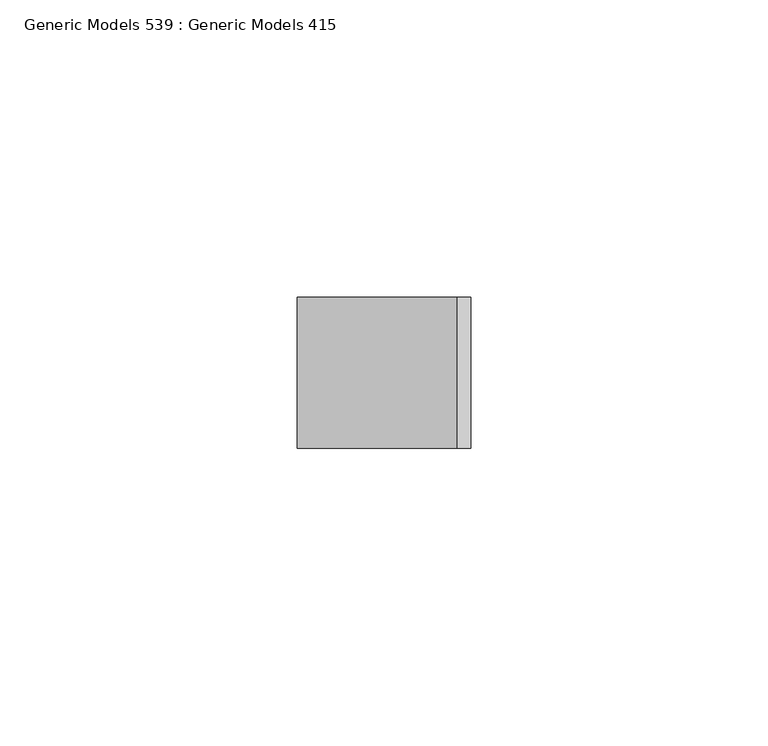
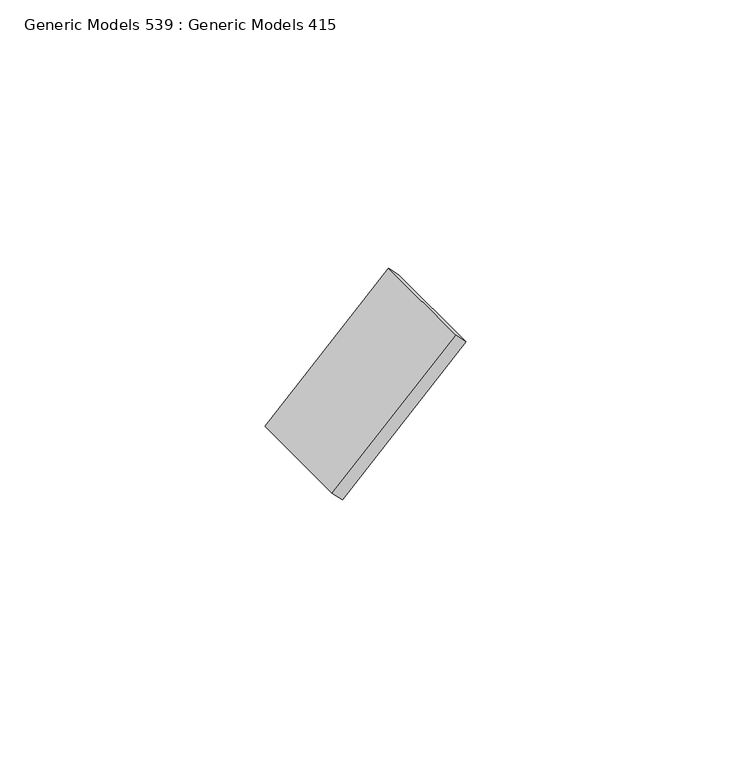
"""IFC4 building model written with IfcOpenShell, lengths in millimetres: proxy geometry, Generic Models 539 : Generic Models 415."""

import ifcopenshell
import ifcopenshell.guid

model = None  # the IFC model being written
_history = None  # IfcOwnerHistory: only IFC2X3 demands one
_inside = {}  # id of a spatial element -> (the spatial element, [elements in it])
_under = {}  # id of a project, library or spatial element -> (it, [spatial elements below it])
_declared = {}  # id of a project -> (the project, [libraries it declares])
_typed = {}  # id of a type object -> (the type object, [elements of that type])
_made_of = {}  # id of a material, layer set ... -> (it, [elements and type objects made of it])


def new_model(schema):
    """Start an empty IFC model of exactly this schema.

    Asked for "IFC4X3", IfcOpenShell would pick the latest addendum, in which some entities
    have other attributes; the version numbers below select the first issue.
    IFC2X3 requires an IfcOwnerHistory on every rooted entity: one is made here for all.
    """
    global model, _history
    if schema == "IFC4X3":
        model = ifcopenshell.file(schema_version=(4, 3, 0, 0))
    else:
        model = ifcopenshell.file(schema=schema)
    _inside.clear()
    _under.clear()
    _declared.clear()
    _typed.clear()
    _made_of.clear()
    _history = None
    if model.schema == "IFC2X3":
        org = make("IfcOrganization", Name="unknown")
        user = make(
            "IfcPersonAndOrganization",
            ThePerson=make("IfcPerson", FamilyName="unknown"),
            TheOrganization=org,
        )
        app = make(
            "IfcApplication",
            ApplicationDeveloper=org,
            Version="unknown",
            ApplicationFullName="unknown",
            ApplicationIdentifier="unknown",
        )
        _history = make(
            "IfcOwnerHistory",
            OwningUser=user,
            OwningApplication=app,
            ChangeAction="ADDED",
            CreationDate=0,
        )
    return model


def make(cls, **values):
    """One entity of the class cls with the attributes given. An attribute that is None is left unset."""
    return model.create_entity(
        cls, **{name: value for name, value in values.items() if value is not None}
    )


def rooted(cls, **values):
    """An entity with a GlobalId (a new one), such as an element, a storey or a relation."""
    return make(cls, GlobalId=ifcopenshell.guid.new(), OwnerHistory=_history, **values)


def si_unit(unit_type, name, prefix=None):
    """IfcSIUnit, for example si_unit("LENGTHUNIT", "METRE", prefix="MILLI")."""
    return make("IfcSIUnit", UnitType=unit_type, Prefix=prefix, Name=name)


def assignment(units):
    """IfcUnitAssignment: the units of a project."""
    return None if units is None else make("IfcUnitAssignment", Units=units)


def point(xyz):
    """IfcCartesianPoint."""
    return None if xyz is None else make("IfcCartesianPoint", Coordinates=xyz)


def direction(xyz):
    """IfcDirection."""
    return None if xyz is None else make("IfcDirection", DirectionRatios=xyz)


def frame(location, z_axis=None, x_axis=None):
    """IfcAxis2Placement3D, a coordinate frame: its origin and axes. An axis left out is left unset."""
    return make(
        "IfcAxis2Placement3D",
        Location=point(location),
        Axis=direction(z_axis),
        RefDirection=direction(x_axis),
    )


def origin():
    """The frame at (0, 0, 0) with its axes left unset."""
    return frame((0.0, 0.0, 0.0))


def place(relative_to, where):
    """IfcLocalPlacement: puts the frame where relative to a parent placement (None: the world)."""
    return make(
        "IfcLocalPlacement", PlacementRelTo=relative_to, RelativePlacement=where
    )


def context(
    kind, dimensions, precision=None, world=None, true_north=None, identifier=None
):
    """IfcGeometricRepresentationContext, for example the 3D "Model" context."""
    return make(
        "IfcGeometricRepresentationContext",
        ContextIdentifier=identifier,
        ContextType=kind,
        CoordinateSpaceDimension=dimensions,
        Precision=precision,
        WorldCoordinateSystem=world,
        TrueNorth=true_north,
    )


def project(units=None, contexts=None):
    """IfcProject with its units and contexts."""
    return rooted(
        "IfcProject",
        Name="project",
        RepresentationContexts=contexts,
        UnitsInContext=assignment(units),
    )


def spatial(cls, under=None, at=None, **own):
    """A site, building, storey or space (cls), placed at a placement, below another one or the project."""
    s = rooted(cls, ObjectPlacement=at, **own)
    if under is not None:
        _under.setdefault(under.id(), (under, []))[1].append(s)
    return s


def polyline(points):
    """IfcPolyline through the points."""
    return make("IfcPolyline", Points=[point(p) for p in points])


def outline(outer, holes=None, kind="AREA"):
    """IfcArbitraryClosedProfileDef: a profile drawn as a closed curve; with holes, ...WithVoids."""
    if holes is None:
        return make("IfcArbitraryClosedProfileDef", ProfileType=kind, OuterCurve=outer)
    return make(
        "IfcArbitraryProfileDefWithVoids",
        ProfileType=kind,
        OuterCurve=outer,
        InnerCurves=holes,
    )


def extrude(swept, where, along, depth):
    """IfcExtrudedAreaSolid: the profile swept, set in the frame where, extruded along a direction by depth."""
    return make(
        "IfcExtrudedAreaSolid",
        SweptArea=swept,
        Position=where,
        ExtrudedDirection=direction(along),
        Depth=depth,
    )


def shape(context_of_items, identifier, shape_type, items):
    """IfcShapeRepresentation: the items that make up one representation, for example the "Body"."""
    return make(
        "IfcShapeRepresentation",
        ContextOfItems=context_of_items,
        RepresentationIdentifier=identifier,
        RepresentationType=shape_type,
        Items=items,
    )


def source(mapping_origin, context_of_items, identifier, shape_type, items):
    """IfcRepresentationMap: a shape defined once, which mapped items show again and again."""
    return make(
        "IfcRepresentationMap",
        MappingOrigin=mapping_origin,
        MappedRepresentation=shape(context_of_items, identifier, shape_type, items),
    )


def transform(
    local_origin,
    x_axis=None,
    y_axis=None,
    z_axis=None,
    scale=None,
    scale2=None,
    scale3=None,
    uniform=True,
):
    """IfcCartesianTransformationOperator3D, or its non-uniform kind. x_axis, y_axis, z_axis: its Axis1, 2, 3."""
    if uniform:
        return make(
            "IfcCartesianTransformationOperator3D",
            Axis1=direction(x_axis),
            Axis2=direction(y_axis),
            LocalOrigin=point(local_origin),
            Scale=scale,
            Axis3=direction(z_axis),
        )
    return make(
        "IfcCartesianTransformationOperator3DnonUniform",
        Axis1=direction(x_axis),
        Axis2=direction(y_axis),
        LocalOrigin=point(local_origin),
        Scale=scale,
        Axis3=direction(z_axis),
        Scale2=scale2,
        Scale3=scale3,
    )


def mapped(mapping_source, mapping_target):
    """IfcMappedItem: shows the shape of a source again, moved by a transform."""
    return make(
        "IfcMappedItem", MappingSource=mapping_source, MappingTarget=mapping_target
    )


def made_of(thing, what):
    """Note that an element or type object is made of a material, layer set ...; save() writes the relation."""
    if what is not None:
        _made_of.setdefault(what.id(), (what, []))[1].append(thing)
    return thing


def element(
    cls,
    number,
    at=None,
    inside=None,
    cuts=None,
    type_object=None,
    material=None,
    context=None,
    identifier="Body",
    shape_type=None,
    held_by="IfcProductDefinitionShape",
    body=None,
    shapes=None,
    **own,
):
    """One element of the class cls, such as IfcWall. Its Tag is "e" and its number.

    at: its placement. inside: the storey or other place that contains it. cuts: it is an
    opening in that element (IfcRelVoidsElement). A single representation is given by context,
    identifier, shape_type and body (its items); several are given by shapes. held_by: the class
    of the entity that holds the representations. save() writes the other relations.
    """
    e = rooted(cls, Tag="e%d" % number, ObjectPlacement=at, **own)
    if body is not None:
        shapes = [shape(context, identifier, shape_type, body)]
    if shapes is not None:
        e.Representation = make(held_by, Representations=shapes)
    if inside is not None:
        _inside.setdefault(inside.id(), (inside, []))[1].append(e)
    if cuts is not None:
        rooted(
            "IfcRelVoidsElement", RelatingBuildingElement=cuts, RelatedOpeningElement=e
        )
    if type_object is not None:
        _typed.setdefault(type_object.id(), (type_object, []))[1].append(e)
    return made_of(e, material)


def aggregate(whole, parts):
    """IfcRelAggregates: a whole, such as a stair, and the parts it consists of."""
    return rooted("IfcRelAggregates", RelatingObject=whole, RelatedObjects=parts)


def save(model, path):
    """Write the relations noted so far, then the file.

    IfcRelAggregates (storeys below a building ...), IfcRelContainedInSpatialStructure (elements
    in a storey), IfcRelDefinesByType, IfcRelAssociatesMaterial and IfcRelDeclares: one each for
    every whole, place, type object, material and project.
    """
    for whole, parts in _under.values():
        aggregate(whole, parts)
    for where, things in _inside.values():
        rooted(
            "IfcRelContainedInSpatialStructure",
            RelatedElements=things,
            RelatingStructure=where,
        )
    for kind, things in _typed.values():
        rooted("IfcRelDefinesByType", RelatedObjects=things, RelatingType=kind)
    for what, things in _made_of.values():
        rooted("IfcRelAssociatesMaterial", RelatedObjects=things, RelatingMaterial=what)
    for by, libraries in _declared.values():
        rooted("IfcRelDeclares", RelatingContext=by, RelatedDefinitions=libraries)
    model.write(path)


def generic_models_539_generic_models_415_c44daec3(model_context):
    return source(origin(), model_context, "Body", "SweptSolid", [
        extrude(outline(polyline([(0.0, -3.175), (0.0, 0.0), (25.4, 0.0), (25.4, -3.175), (0.0, -3.175)])), frame((7848.0411784, 4501.3863946, 125067.3849742), z_axis=(0.7071067811867181, 0.0, 0.707106781186377), x_axis=(0.0, -1.0, 0.0)), (0.0, 0.0, 1.0), 38.1),
    ])


if __name__ == "__main__":
    model = new_model("IFC4")
    model_context = context("Model", 3, world=origin())
    ifc_project = project(units=[si_unit("LENGTHUNIT", "METRE", prefix="MILLI")], contexts=[model_context])
    site = spatial("IfcSite", under=ifc_project)
    building = spatial("IfcBuilding", under=site)
    placement = place(None, origin())
    generic_models_539_generic_models_415_shape = generic_models_539_generic_models_415_c44daec3(model_context)
    element("IfcBuildingElementProxy", 1, Name="Generic Models 539 : Generic Models 415", ObjectType="Generic Models 539 : Generic Models 415", at=placement, inside=building, context=model_context, shape_type="MappedRepresentation", body=[
        mapped(generic_models_539_generic_models_415_shape, transform((0.0, 0.0, 0.0), x_axis=(1.0, 0.0, 0.0), y_axis=(0.0, 1.0, 0.0), z_axis=(0.0, 0.0, 1.0))),
    ])
    save(model, "model.ifc")

# Revit data of these elements
# Element 1 (IfcBuildingElementProxy, "Generic Models 539 : Generic Models 415")
#   Materials on its faces: "_WELDED STEEL TABS FOR LOUVER ATTACHMENT"
# Materials
#   "_WELDED STEEL TABS FOR LOUVER ATTACHMENT": class "Metal", colour RGB 199 199 199, transparency 0, Description = "Structural steel 50ksi", Cost = 0
